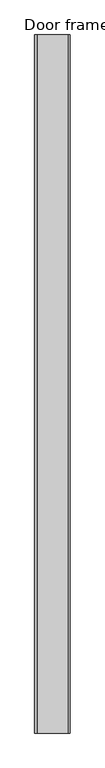
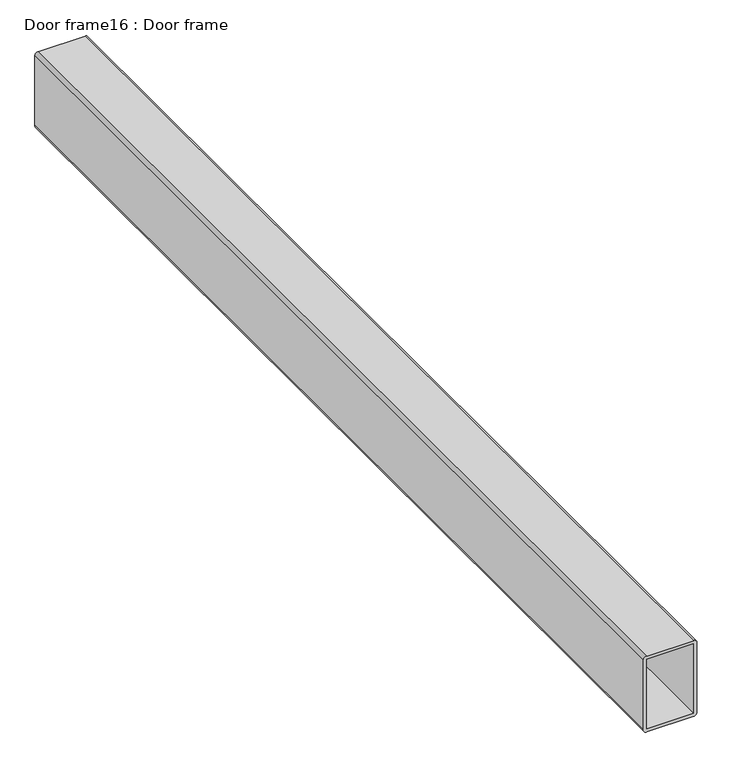
"""IFC4 building model written with IfcOpenShell, lengths in millimetres: proxy geometry, Door frame16 : Door frame."""

from ifc_helpers import new_model, si_unit, point, frame, frame_2d, origin, place, context, project, spatial, polyline, circle_curve, trimmed, segment, composite_curve, outline, extrude, source, transform, mapped, element, save


def door_frame16_door_frame_b90efb81(model_context):
    return source(origin(), model_context, "Body", "SweptSolid", [
        extrude(outline(composite_curve([segment(polyline([(34855.8775473, -8390.3106967), (34855.8775473, -8301.4106967)]), True, "CONTINUOUS"), segment(trimmed(circle_curve(frame_2d((34862.2275473, -8301.4106967)), 6.35), [point((34855.8775473, -8301.4106967))], [point((34862.2275473, -8295.0606967))], False, "CARTESIAN"), True, "CONTINUOUS"), segment(polyline([(34862.2275473, -8295.0606967), (35001.9275473, -8295.0606967)]), True, "CONTINUOUS"), segment(trimmed(circle_curve(frame_2d((35001.9275473, -8301.4106967)), 6.35), [point((35001.9275473, -8295.0606967))], [point((35008.2775473, -8301.4106967))], False, "CARTESIAN"), True, "CONTINUOUS"), segment(polyline([(35008.2775473, -8301.4106967), (35008.2775473, -8390.3106967)]), True, "CONTINUOUS"), segment(trimmed(circle_curve(frame_2d((35001.9275473, -8390.3106967)), 6.35), [point((35008.2775473, -8390.3106967))], [point((35001.9275473, -8396.6606967))], False, "CARTESIAN"), True, "CONTINUOUS"), segment(polyline([(35001.9275473, -8396.6606967), (34862.2275473, -8396.6606967)]), True, "CONTINUOUS"), segment(trimmed(circle_curve(frame_2d((34862.2275473, -8390.3106967)), 6.35), [point((34862.2275473, -8396.6606967))], [point((34855.8775473, -8390.3106967))], False, "CARTESIAN"), True, "CONTINUOUS")], self_intersect=False), holes=[polyline([(35001.7775473, -8301.5606967), (34862.3775473, -8301.5606967), (34862.3775473, -8390.1606967), (35001.7775473, -8390.1606967), (35001.7775473, -8301.5606967)])]), frame((0.0, 4540.4513244, 0.0), z_axis=(0.0, 1.0, 0.0), x_axis=(0.0, 0.0, 1.0)), (0.0, 0.0, 1.0), 2000.0),
    ])


if __name__ == "__main__":
    model = new_model("IFC4")
    model_context = context("Model", 3, world=origin())
    ifc_project = project(units=[si_unit("LENGTHUNIT", "METRE", prefix="MILLI")], contexts=[model_context])
    site = spatial("IfcSite", under=ifc_project)
    building = spatial("IfcBuilding", under=site)
    placement = place(None, origin())
    door_frame16_door_frame_shape = door_frame16_door_frame_b90efb81(model_context)
    element("IfcBuildingElementProxy", 1, Name="Door frame16 : Door frame", ObjectType="Door frame16 : Door frame", at=placement, inside=building, context=model_context, shape_type="MappedRepresentation", body=[
        mapped(door_frame16_door_frame_shape, transform((0.0, 0.0, 0.0), x_axis=(1.0, 0.0, 0.0), y_axis=(0.0, 1.0, 0.0), z_axis=(0.0, 0.0, 1.0))),
    ])
    save(model, "model.ifc")

# Revit data of these elements
# Type "Door frame16 : Door frame"
#   NameOverride = "Door frame"
# Element 1 (IfcBuildingElementProxy, "Door frame16 : Door frame")
#   Materials on its faces: "DOOR FRAME: TUBE STEEL PROFILE - METALIZED, PRIMED & PAINTED (COLOR PER ARCHITECT)"
# Materials
#   "DOOR FRAME: TUBE STEEL PROFILE - METALIZED, PRIMED & PAINTED (COLOR PER ARCHITECT)": class "Unassigned", colour RGB 128 128 128, transparency 0, Cost = 0
